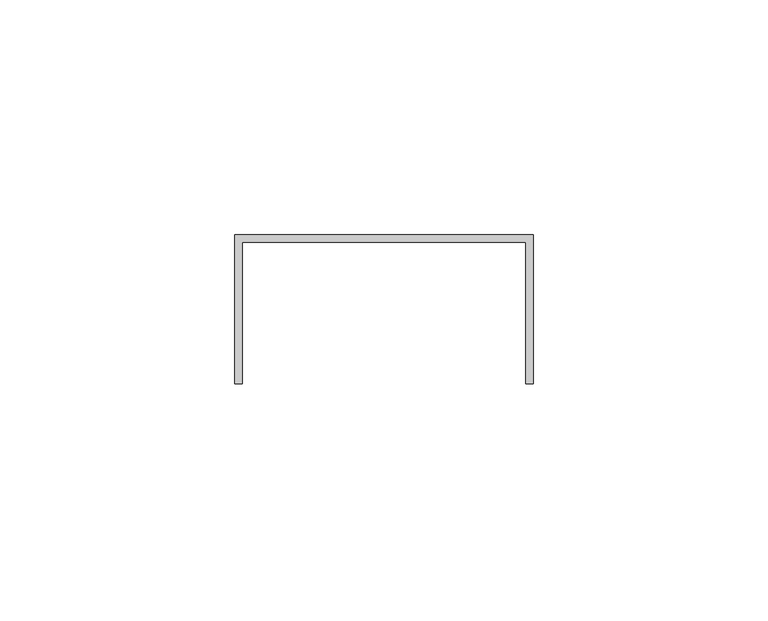
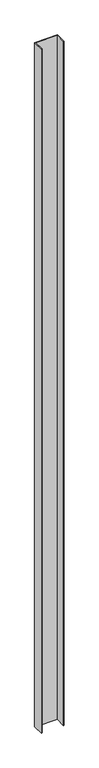
"""IFC4 building model written with IfcOpenShell, lengths in millimetres: proxy geometry, Generic Models 7:Generic Models 1:3:Generic Models 1:3 : Generic Models 7:Generic Models 1:305549:3:Generic Models 1:3:Generic Models 1:3 : Generic Models 7:Generic Models 1:305549:3 : Generic Models 7:Generic Models 1:3:Generic Models 1:3 : Generic Models 7:Generic Models 1:305549:301244:26 : Generic Models 7:Generic Models 1:3:Generic Models 1:3 : Generic Models 7:Generic Models 1:305549:3:Generic Models 1:3:Generic Models 1:3 : Generic Models 7:Generic Models 1:305549:3 : Generic Models 7:Generic Models 1:3:Generic Models 1:3 : Generic Models 7:Generic Models 1:305549:301244:308848."""

from ifc_helpers import new_model, si_unit, frame, origin, place, context, project, spatial, polyline, outline, extrude, source, transform, mapped, element, save


def generic_models_65c3a93f(model_context):
    return source(origin(), model_context, "Body", "SweptSolid", [
        extrude(outline(polyline([(560340.2617239, -572599.8913841), (560340.2617239, -572631.6413841), (560338.6742239, -572631.6413841), (560338.6742239, -572601.4788841), (560278.3492239, -572601.4788841), (560278.3492239, -572631.6413841), (560276.7617239, -572631.6413841), (560276.7617239, -572599.8913841), (560340.2617239, -572599.8913841)])), frame((0.0, 0.0, 4133.81326), z_axis=(0.0, 0.0, 1.0), x_axis=(1.0, 0.0, 0.0)), (0.0, 0.0, 1.0), 2000.28674),
    ])


if __name__ == "__main__":
    model = new_model("IFC4")
    model_context = context("Model", 3, world=origin())
    ifc_project = project(units=[si_unit("LENGTHUNIT", "METRE", prefix="MILLI")], contexts=[model_context])
    site = spatial("IfcSite", under=ifc_project)
    building = spatial("IfcBuilding", under=site)
    placement = place(None, origin())
    generic_models_shape = generic_models_65c3a93f(model_context)
    element("IfcBuildingElementProxy", 1, Name="Generic Models 7:Generic Models 1:3:Generic Models 1:3 : Generic Models 7:Generic Models 1:305549:3:Generic Models 1:3:Generic Models 1:3 : Generic Models 7:Generic Models 1:305549:3 : Generic Models 7:Generic Models 1:3:Generic Models 1:3 : Generic Models 7:Generic Models 1:305549:301244:26 : Generic Models 7:Generic Models 1:3:Generic Models 1:3 : Generic Models 7:Generic Models 1:305549:3:Generic Models 1:3:Generic Models 1:3 : Generic Models 7:Generic Models 1:305549:3 : Generic Models 7:Generic Models 1:3:Generic Models 1:3 : Generic Models 7:Generic Models 1:305549:301244:308848", ObjectType="Generic Models 7:Generic Models 1:3:Generic Models 1:3 : Generic Models 7:Generic Models 1:305549:3:Generic Models 1:3:Generic Models 1:3 : Generic Models 7:Generic Models 1:305549:3 : Generic Models 7:Generic Models 1:3:Generic Models 1:3 : Generic Models 7:Generic Models 1:305549:301244:26 : Generic Models 7:Generic Models 1:3:Generic Models 1:3 : Generic Models 7:Generic Models 1:305549:3:Generic Models 1:3:Generic Models 1:3 : Generic Models 7:Generic Models 1:305549:3 : Generic Models 7:Generic Models 1:3:Generic Models 1:3 : Generic Models 7:Generic Models 1:305549:301244:308848", at=placement, inside=building, context=model_context, shape_type="MappedRepresentation", body=[
        mapped(generic_models_shape, transform((0.0, 0.0, 0.0), x_axis=(1.0, 0.0, 0.0), y_axis=(0.0, 1.0, 0.0), z_axis=(0.0, 0.0, 1.0))),
    ])
    save(model, "model.ifc")

# Revit data of these elements
# Type "Generic Models 7:Generic Models 1:3:Generic Models 1:3 : Generic Models 7:Generic Models 1:305549:3:Generic Models 1:3:Generic Models 1:3 : Generic Models 7:Generic Models 1:305549:3 : Generic Models 7:Generic Models 1:3:Generic Models 1:3 : Generic Models 7:Generic Models 1:305549:301244:26 : Generic Models 7:Generic Models 1:3:Generic Models 1:3 : Generic Models 7:Generic Models 1:305549:3:Generic Models 1:3:Generic Models 1:3 : Generic Models 7:Generic Models 1:305549:3 : Generic Models 7:Generic Models 1:3:Generic Models 1:3 : Generic Models 7:Generic Models 1:305549:301244:308848"
#   NameOverride = "Generic Models 7:Generic Models 1:3:Generic Models 1:3 : Generic Models 7:Generic Models 1:305549:3:Generic Models 1:3:Generic Models 1:3 : Generic Models 7:Generic Models 1:305549:3 : Generic Models 7:Generic Models 1:3:Generic Models 1:3 : Generic Models 7:Generic Models 1:305549:301244:308848"
#   ObjectTypeOverride = "Generic Models 1:3:Generic Models 1:3 : Generic Models 7:Generic Models 1:305549:3 : Generic Models 7:Generic Models 1:3:Generic Models 1:3 : Generic Models 7:Generic Models 1:305549:301244"
#   Reference = "Generic Models 1"
#   Tag = "308848"
# Element 1 (IfcBuildingElementProxy, "Generic Models 7:Generic Models 1:3:Generic Models 1:3 : Generic Models 7:Generic Models 1:305549:3:Generic Models 1:3:Generic Models 1:3 : Generic Models 7:Generic Models 1:305549:3 : Generic Models 7:Generic Models 1:3:Generic Models 1:3 : Generic Models 7:Generic Models 1:305549:301244:26 : Generic Models 7:Generic Models 1:3:Generic Models 1:3 : Generic Models 7:Generic Models 1:305549:3:Generic Models 1:3:Generic Models 1:3 : Generic Models 7:Generic Models 1:305549:3 : Generic Models 7:Generic Models 1:3:Generic Models 1:3 : Generic Models 7:Generic Models 1:305549:301244:308848")
#   Materials on its faces: "GALVANIZED U-CHANNEL (250T125-33)"
# Materials
#   "GALVANIZED U-CHANNEL (250T125-33)": class "Unassigned", colour RGB 202 201 200, transparency 0, Keynote = "M05451300.02", Cost = 0
